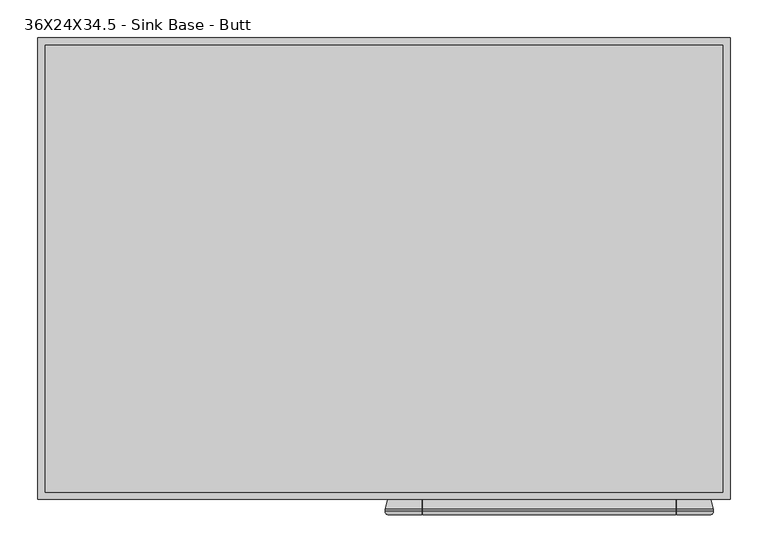
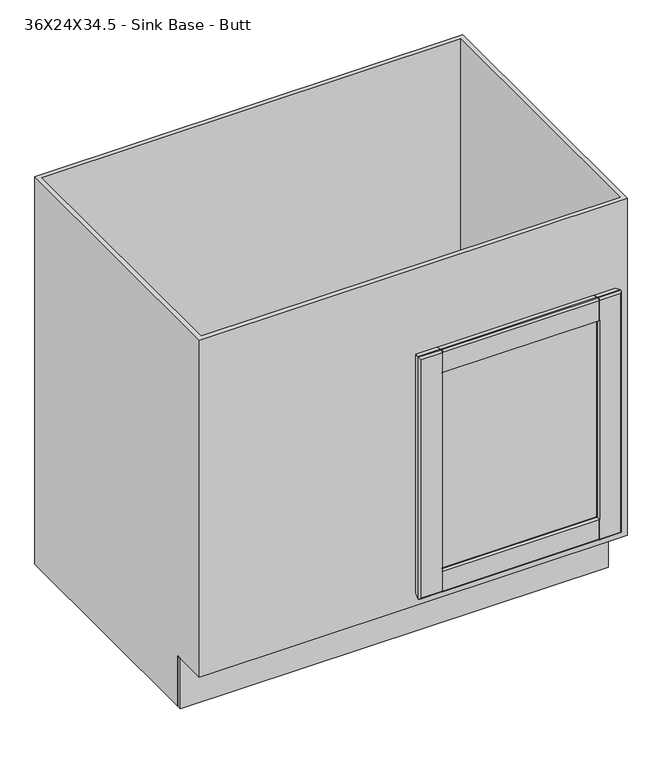
"""IFC4 building model written with IfcOpenShell, lengths in millimetres: furniture geometry, Cabinet-Base-Merillat-Double_Door-Marlin : 36X24X34.5 - Sink Base - Butt."""

import ifcopenshell
import ifcopenshell.guid

model = None  # the IFC model being written
_history = None  # IfcOwnerHistory: only IFC2X3 demands one
_inside = {}  # id of a spatial element -> (the spatial element, [elements in it])
_under = {}  # id of a project, library or spatial element -> (it, [spatial elements below it])
_declared = {}  # id of a project -> (the project, [libraries it declares])
_typed = {}  # id of a type object -> (the type object, [elements of that type])
_made_of = {}  # id of a material, layer set ... -> (it, [elements and type objects made of it])


def new_model(schema):
    """Start an empty IFC model of exactly this schema.

    Asked for "IFC4X3", IfcOpenShell would pick the latest addendum, in which some entities
    have other attributes; the version numbers below select the first issue.
    IFC2X3 requires an IfcOwnerHistory on every rooted entity: one is made here for all.
    """
    global model, _history
    if schema == "IFC4X3":
        model = ifcopenshell.file(schema_version=(4, 3, 0, 0))
    else:
        model = ifcopenshell.file(schema=schema)
    _inside.clear()
    _under.clear()
    _declared.clear()
    _typed.clear()
    _made_of.clear()
    _history = None
    if model.schema == "IFC2X3":
        org = make("IfcOrganization", Name="unknown")
        user = make(
            "IfcPersonAndOrganization",
            ThePerson=make("IfcPerson", FamilyName="unknown"),
            TheOrganization=org,
        )
        app = make(
            "IfcApplication",
            ApplicationDeveloper=org,
            Version="unknown",
            ApplicationFullName="unknown",
            ApplicationIdentifier="unknown",
        )
        _history = make(
            "IfcOwnerHistory",
            OwningUser=user,
            OwningApplication=app,
            ChangeAction="ADDED",
            CreationDate=0,
        )
    return model


def make(cls, **values):
    """One entity of the class cls with the attributes given. An attribute that is None is left unset."""
    return model.create_entity(
        cls, **{name: value for name, value in values.items() if value is not None}
    )


def rooted(cls, **values):
    """An entity with a GlobalId (a new one), such as an element, a storey or a relation."""
    return make(cls, GlobalId=ifcopenshell.guid.new(), OwnerHistory=_history, **values)


def si_unit(unit_type, name, prefix=None):
    """IfcSIUnit, for example si_unit("LENGTHUNIT", "METRE", prefix="MILLI")."""
    return make("IfcSIUnit", UnitType=unit_type, Prefix=prefix, Name=name)


def assignment(units):
    """IfcUnitAssignment: the units of a project."""
    return None if units is None else make("IfcUnitAssignment", Units=units)


def point(xyz):
    """IfcCartesianPoint."""
    return None if xyz is None else make("IfcCartesianPoint", Coordinates=xyz)


def direction(xyz):
    """IfcDirection."""
    return None if xyz is None else make("IfcDirection", DirectionRatios=xyz)


def frame(location, z_axis=None, x_axis=None):
    """IfcAxis2Placement3D, a coordinate frame: its origin and axes. An axis left out is left unset."""
    return make(
        "IfcAxis2Placement3D",
        Location=point(location),
        Axis=direction(z_axis),
        RefDirection=direction(x_axis),
    )


def origin():
    """The frame at (0, 0, 0) with its axes left unset."""
    return frame((0.0, 0.0, 0.0))


def origin_with_axes():
    """The frame at (0, 0, 0) with the z axis (0, 0, 1) and the x axis (1, 0, 0) written out."""
    return frame((0.0, 0.0, 0.0), z_axis=(0.0, 0.0, 1.0), x_axis=(1.0, 0.0, 0.0))


def place(relative_to, where):
    """IfcLocalPlacement: puts the frame where relative to a parent placement (None: the world)."""
    return make(
        "IfcLocalPlacement", PlacementRelTo=relative_to, RelativePlacement=where
    )


def context(
    kind, dimensions, precision=None, world=None, true_north=None, identifier=None
):
    """IfcGeometricRepresentationContext, for example the 3D "Model" context."""
    return make(
        "IfcGeometricRepresentationContext",
        ContextIdentifier=identifier,
        ContextType=kind,
        CoordinateSpaceDimension=dimensions,
        Precision=precision,
        WorldCoordinateSystem=world,
        TrueNorth=true_north,
    )


def project(units=None, contexts=None):
    """IfcProject with its units and contexts."""
    return rooted(
        "IfcProject",
        Name="project",
        RepresentationContexts=contexts,
        UnitsInContext=assignment(units),
    )


def spatial(cls, under=None, at=None, **own):
    """A site, building, storey or space (cls), placed at a placement, below another one or the project."""
    s = rooted(cls, ObjectPlacement=at, **own)
    if under is not None:
        _under.setdefault(under.id(), (under, []))[1].append(s)
    return s


def polyline(points):
    """IfcPolyline through the points."""
    return make("IfcPolyline", Points=[point(p) for p in points])


def circle_curve(where, radius):
    """IfcCircle in the frame where."""
    return make("IfcCircle", Position=where, Radius=radius)


def ellipse_curve(where, semi_axis1, semi_axis2):
    """IfcEllipse in the frame where."""
    return make(
        "IfcEllipse", Position=where, SemiAxis1=semi_axis1, SemiAxis2=semi_axis2
    )


def outline(outer, holes=None, kind="AREA"):
    """IfcArbitraryClosedProfileDef: a profile drawn as a closed curve; with holes, ...WithVoids."""
    if holes is None:
        return make("IfcArbitraryClosedProfileDef", ProfileType=kind, OuterCurve=outer)
    return make(
        "IfcArbitraryProfileDefWithVoids",
        ProfileType=kind,
        OuterCurve=outer,
        InnerCurves=holes,
    )


def extrude(swept, where, along, depth):
    """IfcExtrudedAreaSolid: the profile swept, set in the frame where, extruded along a direction by depth."""
    return make(
        "IfcExtrudedAreaSolid",
        SweptArea=swept,
        Position=where,
        ExtrudedDirection=direction(along),
        Depth=depth,
    )


def faces_of(points, faces, orient=None, outer=None):
    """IfcFace entities. A face is a list of loops; a loop is a list of indices into points, from 0.

    orient and outer hold one flag for each loop. By default every Orientation is true, the
    first loop of a face is its IfcFaceOuterBound and the others are IfcFaceBound.
    """
    made = []
    for i, loops in enumerate(faces):
        bounds = []
        for j, loop in enumerate(loops):
            is_outer = j == 0 if outer is None else outer[i][j]
            bounds.append(
                make(
                    "IfcFaceOuterBound" if is_outer else "IfcFaceBound",
                    Bound=make("IfcPolyLoop", Polygon=[points[k] for k in loop]),
                    Orientation=True if orient is None else orient[i][j],
                )
            )
        made.append(make("IfcFace", Bounds=bounds))
    return made


def faceted_brep(points, faces, orient=None, outer=None, voids=None):
    """IfcFacetedBrep: a solid bounded by flat faces; with voids (closed shells), ...WithVoids."""
    shared = [point(p) for p in points]
    hull = make("IfcClosedShell", CfsFaces=faces_of(shared, faces, orient, outer))
    if voids is None:
        return make("IfcFacetedBrep", Outer=hull)
    return make(
        "IfcFacetedBrepWithVoids",
        Outer=hull,
        Voids=[
            make(cls, CfsFaces=faces_of(shared, fs, o, b)) for cls, fs, o, b in voids
        ],
    )


def shape(context_of_items, identifier, shape_type, items):
    """IfcShapeRepresentation: the items that make up one representation, for example the "Body"."""
    return make(
        "IfcShapeRepresentation",
        ContextOfItems=context_of_items,
        RepresentationIdentifier=identifier,
        RepresentationType=shape_type,
        Items=items,
    )


def source(mapping_origin, context_of_items, identifier, shape_type, items):
    """IfcRepresentationMap: a shape defined once, which mapped items show again and again."""
    return make(
        "IfcRepresentationMap",
        MappingOrigin=mapping_origin,
        MappedRepresentation=shape(context_of_items, identifier, shape_type, items),
    )


def transform(
    local_origin,
    x_axis=None,
    y_axis=None,
    z_axis=None,
    scale=None,
    scale2=None,
    scale3=None,
    uniform=True,
):
    """IfcCartesianTransformationOperator3D, or its non-uniform kind. x_axis, y_axis, z_axis: its Axis1, 2, 3."""
    if uniform:
        return make(
            "IfcCartesianTransformationOperator3D",
            Axis1=direction(x_axis),
            Axis2=direction(y_axis),
            LocalOrigin=point(local_origin),
            Scale=scale,
            Axis3=direction(z_axis),
        )
    return make(
        "IfcCartesianTransformationOperator3DnonUniform",
        Axis1=direction(x_axis),
        Axis2=direction(y_axis),
        LocalOrigin=point(local_origin),
        Scale=scale,
        Axis3=direction(z_axis),
        Scale2=scale2,
        Scale3=scale3,
    )


def mapped(mapping_source, mapping_target):
    """IfcMappedItem: shows the shape of a source again, moved by a transform."""
    return make(
        "IfcMappedItem", MappingSource=mapping_source, MappingTarget=mapping_target
    )


def made_of(thing, what):
    """Note that an element or type object is made of a material, layer set ...; save() writes the relation."""
    if what is not None:
        _made_of.setdefault(what.id(), (what, []))[1].append(thing)
    return thing


def element(
    cls,
    number,
    at=None,
    inside=None,
    cuts=None,
    type_object=None,
    material=None,
    context=None,
    identifier="Body",
    shape_type=None,
    held_by="IfcProductDefinitionShape",
    body=None,
    shapes=None,
    **own,
):
    """One element of the class cls, such as IfcWall. Its Tag is "e" and its number.

    at: its placement. inside: the storey or other place that contains it. cuts: it is an
    opening in that element (IfcRelVoidsElement). A single representation is given by context,
    identifier, shape_type and body (its items); several are given by shapes. held_by: the class
    of the entity that holds the representations. save() writes the other relations.
    """
    e = rooted(cls, Tag="e%d" % number, ObjectPlacement=at, **own)
    if body is not None:
        shapes = [shape(context, identifier, shape_type, body)]
    if shapes is not None:
        e.Representation = make(held_by, Representations=shapes)
    if inside is not None:
        _inside.setdefault(inside.id(), (inside, []))[1].append(e)
    if cuts is not None:
        rooted(
            "IfcRelVoidsElement", RelatingBuildingElement=cuts, RelatedOpeningElement=e
        )
    if type_object is not None:
        _typed.setdefault(type_object.id(), (type_object, []))[1].append(e)
    return made_of(e, material)


def aggregate(whole, parts):
    """IfcRelAggregates: a whole, such as a stair, and the parts it consists of."""
    return rooted("IfcRelAggregates", RelatingObject=whole, RelatedObjects=parts)


def save(model, path):
    """Write the relations noted so far, then the file.

    IfcRelAggregates (storeys below a building ...), IfcRelContainedInSpatialStructure (elements
    in a storey), IfcRelDefinesByType, IfcRelAssociatesMaterial and IfcRelDeclares: one each for
    every whole, place, type object, material and project.
    """
    for whole, parts in _under.values():
        aggregate(whole, parts)
    for where, things in _inside.values():
        rooted(
            "IfcRelContainedInSpatialStructure",
            RelatedElements=things,
            RelatingStructure=where,
        )
    for kind, things in _typed.values():
        rooted("IfcRelDefinesByType", RelatedObjects=things, RelatingType=kind)
    for what, things in _made_of.values():
        rooted("IfcRelAssociatesMaterial", RelatedObjects=things, RelatingMaterial=what)
    for by, libraries in _declared.values():
        rooted("IfcRelDeclares", RelatingContext=by, RelatedDefinitions=libraries)
    model.write(path)


def plane_surface(at):
    """IfcPlane: the flat surface through the origin of the frame at, square to its z axis."""
    return make("IfcPlane", Position=at)


def cylinder_surface(at, radius):
    """IfcCylindricalSurface: all points at the distance radius from the z axis of the frame at."""
    return make("IfcCylindricalSurface", Position=at, Radius=radius)


def advanced_brep(points, edges, surfaces, faces):
    """IfcAdvancedBrep: a solid bounded by faces that lie on surfaces and meet in shared edges.

    An edge is (start, end): straight between two places in points (the first is 0);
    or (start, end, curve); or (start, end, curve, False) where it runs against its curve.
    A face is (place in surfaces, loops), or (place, loops, False) where it looks against
    its surface's normal. A loop lists edges by number (the first is 1), with a minus sign
    where the edge is run from its end to its start. The first loop is the outer one.
    """
    corners = [point(p) for p in points]
    vertices = [make("IfcVertexPoint", VertexGeometry=c) for c in corners]
    made = []
    for start, end, *more in edges:
        made.append(
            make(
                "IfcEdgeCurve",
                EdgeStart=vertices[start],
                EdgeEnd=vertices[end],
                EdgeGeometry=more[0] if more else make("IfcPolyline", Points=[corners[start], corners[end]]),
                SameSense=more[1] if len(more) > 1 else True,
            )
        )
    hull = []
    for where, loops, *sense in faces:
        bounds = []
        for j, loop in enumerate(loops):
            ring = [make("IfcOrientedEdge", EdgeElement=made[abs(k) - 1], Orientation=k > 0) for k in loop]
            bounds.append(
                make(
                    "IfcFaceOuterBound" if j == 0 else "IfcFaceBound",
                    Bound=make("IfcEdgeLoop", EdgeList=ring),
                    Orientation=True,
                )
            )
        hull.append(make("IfcAdvancedFace", Bounds=bounds, FaceSurface=surfaces[where], SameSense=sense[0] if sense else True))
    return make("IfcAdvancedBrep", Outer=make("IfcClosedShell", CfsFaces=hull))


def furniture_36x24x34_5_sink_base_butt_f9e5757f(model_context):
    return source(origin(), model_context, "Body", "SolidModel", [
        advanced_brep(
        [(453.7127049, -625.4496, 685.8), (450.6162124, -629.92, 682.7035075), (450.6162124, -629.92, 142.7964925), (453.7127049, -625.4496, 139.7), (453.7127049, -622.681, 139.7), (453.7127049, -622.681, 685.8), (450.2075049, -609.6, 143.2052), (450.2075049, -609.6, 682.2948), (405.5115422, -609.6, 637.5988372), (405.5115422, -609.6, 187.9011628), (405.1414105, -610.39375, 188.2712945), (403.0602514, -614.85681, 190.3524535), (403.0602514, -614.85681, 635.1475465), (405.1414105, -610.39375, 637.2287055), (404.4600209, -617.0969093, 188.952684), (404.4600209, -617.0969093, 636.547316), (418.7877049, -617.347, 174.625), (418.7877049, -617.347, 650.875), (418.7877049, -622.173, 174.625), (418.7877049, -622.173, 650.875), (404.4600209, -622.4230907, 188.952684), (404.4600209, -622.4230907, 636.547316), (403.0602514, -624.66319, 190.3524535), (403.0602514, -624.66319, 635.1475465), (405.1414105, -629.12625, 188.2712945), (405.5086747, -629.9138508, 187.9040302), (405.5115422, -629.92, 637.5988372), (405.1414105, -629.12625, 637.2287055), (405.5086747, -629.92, 142.7964925), (405.5086747, -625.4496, 139.7), (23.4216974, -629.92, 142.7964925), (20.3252049, -625.4496, 139.7), (68.4894236, -625.4496, 139.7), (68.4894236, -629.92, 142.7964925), (403.9211747, -625.4496, 139.7), (403.9211747, -629.92, 142.7964925), (70.0769236, -629.92, 142.7964925), (70.0769236, -625.4496, 139.7), (405.5086747, -622.681, 139.7), (20.3252049, -622.681, 139.7), (68.4894236, -622.681, 139.7), (403.9211747, -622.681, 139.7), (70.0769236, -622.681, 139.7), (405.5086747, -609.6, 143.2052), (23.8304049, -609.6, 143.2052), (68.4894236, -609.6, 143.2052), (403.9211747, -609.6, 143.2052), (70.0769236, -609.6, 143.2052), (70.9776584, -614.85681, 190.3524535), (403.9211747, -610.39375, 188.2712945), (403.9211747, -609.6, 187.9011628), (70.0769236, -609.6, 187.9011628), (70.0769236, -610.39375, 188.2712945), (68.8964994, -610.39375, 188.2712945), (69.577889, -617.0969093, 188.952684), (55.2502049, -617.347, 174.625), (55.2502049, -622.173, 174.625), (69.577889, -622.4230907, 188.952684), (70.9776584, -624.66319, 190.3524535), (68.8964994, -629.12625, 188.2712945), (70.0769236, -629.12625, 188.2712945), (70.0769236, -629.92, 187.9011628), (403.9211747, -629.92, 187.9011628), (403.9211747, -629.12625, 188.2712945), (23.4216974, -629.92, 682.7035075), (20.3252049, -625.4496, 685.8), (20.3252049, -622.681, 685.8), (23.8304049, -609.6, 682.2948), (68.5263677, -609.6, 187.9011628), (68.5263677, -609.6, 637.5988372), (68.8964994, -610.39375, 637.2287055), (70.9776584, -614.85681, 635.1475465), (69.577889, -617.0969093, 636.547316), (55.2502049, -617.347, 650.875), (55.2502049, -622.173, 650.875), (69.577889, -622.4230907, 636.547316), (70.9776584, -624.66319, 635.1475465), (68.8964994, -629.12625, 637.2287055), (68.5263677, -629.92, 637.5988372), (68.5263677, -629.92, 187.9011628), (68.4894236, -629.92, 682.7035075), (68.4894236, -625.4496, 685.8), (405.5086747, -625.4496, 685.8), (405.5086747, -629.92, 682.7035075), (70.0769236, -625.4496, 685.8), (70.0769236, -629.92, 682.7035075), (403.9211747, -629.92, 682.7035075), (403.9211747, -625.4496, 685.8), (68.4894236, -622.681, 685.8), (405.5086747, -622.681, 685.8), (70.0769236, -622.681, 685.8), (403.9211747, -622.681, 685.8), (68.4894236, -609.6, 682.2948), (405.5086747, -609.6, 682.2948), (70.0769236, -609.6, 682.2948), (403.9211747, -609.6, 682.2948), (70.0769236, -609.6, 637.5988372), (403.9211747, -609.6, 637.5988372), (70.0769236, -610.39375, 637.2287055), (403.9211747, -610.39375, 637.2287055), (403.9211747, -629.12625, 637.2287055), (403.9211747, -629.92, 637.5988372), (70.0769236, -629.92, 637.5988372), (70.0769236, -629.12625, 637.2287055), (70.0769236, -610.39375, 681.6857412), (70.0769236, -622.7855037, 685.00625), (70.0769236, -625.4496, 685.00625), (70.0769236, -629.12625, 682.5526052), (68.4894236, -629.12625, 637.2287055), (68.4894236, -629.12625, 682.5526052), (68.4894236, -625.4496, 685.00625), (68.4894236, -622.7855037, 685.00625), (68.4894236, -610.39375, 681.6857412), (68.4894236, -610.39375, 637.2287055), (405.5086747, -610.39375, 637.2287055), (405.5086747, -610.39375, 681.6857412), (405.5086747, -622.7855037, 685.00625), (405.5086747, -625.4496, 685.00625), (405.5086747, -629.12625, 682.5526052), (405.5086747, -629.12625, 637.2287055), (403.9211747, -629.12625, 682.5526052), (403.9211747, -625.4496, 685.00625), (403.9211747, -622.7855037, 685.00625), (403.9211747, -610.39375, 681.6857412), (405.5086747, -629.12625, 188.2712945), (405.5086747, -629.12625, 142.9473948), (405.5086747, -625.4496, 140.49375), (405.5086747, -622.7855037, 140.49375), (405.5086747, -610.39375, 143.8142588), (405.5086747, -610.39375, 188.2712945), (403.9211747, -610.39375, 143.8142588), (403.9211747, -622.7855037, 140.49375), (403.9211747, -625.4496, 140.49375), (403.9211747, -629.12625, 142.9473948), (70.0769236, -629.12625, 142.9473948), (70.0769236, -625.4496, 140.49375), (70.0769236, -622.7855037, 140.49375), (70.0769236, -610.39375, 143.8142588), (68.4894236, -629.12625, 188.2712945), (68.4894236, -610.39375, 188.2712945), (68.4894236, -610.39375, 143.8142588), (68.4894236, -622.7855037, 140.49375), (68.4894236, -625.4496, 140.49375), (68.4894236, -629.12625, 142.9473948)],
        [
            (0, 1, ellipse_curve(frame((448.9375049, -625.4496, 681.0248), z_axis=(0.7071067811865475, 0.0, -0.7071067811865475), x_axis=(0.7071067811865474, 0.0, 0.7071067811865476)), 6.7531526, 4.7752)),
            (1, 2),
            (2, 3, ellipse_curve(frame((448.9375049, -625.4496, 144.4752), z_axis=(0.7071067811865475, 0.0, 0.7071067811865475), x_axis=(-0.7071067811865474, 0.0, 0.7071067811865476)), 6.7531526, 4.7752)),
            (3, 0),
            (3, 4),
            (4, 5),
            (5, 0),
            (4, 6),
            (6, 7),
            (7, 5),
            (8, 9),
            (9, 10),
            (10, 11),
            (11, 12),
            (12, 13),
            (13, 8),
            (11, 14, ellipse_curve(frame((404.4875049, -615.5223492, 188.9252), z_axis=(0.7071067811865475, 0.0, 0.7071067811865475), x_axis=(-0.7071067811865474, 0.0, 0.7071067811865476)), 2.2271035, 1.5748)),
            (14, 15),
            (15, 12, ellipse_curve(frame((404.4875049, -615.5223492, 636.5748), z_axis=(0.7071067811865475, 0.0, -0.7071067811865475), x_axis=(0.7071067811865474, 0.0, 0.7071067811865476)), 2.2271035, 1.5748)),
            (14, 16),
            (16, 17),
            (17, 15),
            (16, 18),
            (18, 19),
            (19, 17),
            (18, 20),
            (20, 21),
            (21, 19),
            (20, 22, ellipse_curve(frame((404.4875049, -623.9976508, 188.9252), z_axis=(0.7071067811865475, 0.0, 0.7071067811865475), x_axis=(-0.7071067811865474, 0.0, 0.7071067811865476)), 2.2271035, 1.5748)),
            (22, 23),
            (23, 21, ellipse_curve(frame((404.4875049, -623.9976508, 636.5748), z_axis=(0.7071067811865475, 0.0, -0.7071067811865475), x_axis=(0.7071067811865474, 0.0, 0.7071067811865476)), 2.2271035, 1.5748)),
            (22, 24),
            (24, 25),
            (25, 26),
            (26, 27),
            (27, 23),
            (2, 28),
            (28, 29, circle_curve(frame((405.5086747, -625.4496, 144.4752), z_axis=(1.0, 0.0, 0.0), x_axis=(0.0, 1.0, 0.0)), 4.7752)),
            (29, 3),
            (30, 31, ellipse_curve(frame((25.1004049, -625.4496, 144.4752), z_axis=(0.7071067811865475, 0.0, -0.7071067811865475), x_axis=(0.7071067811865476, 0.0, 0.7071067811865474)), 6.7531526, 4.7752)),
            (31, 32),
            (32, 33, circle_curve(frame((68.4894236, -625.4496, 144.4752), z_axis=(-1.0, 0.0, 0.0), x_axis=(0.0, 1.0, 0.0)), 4.7752)),
            (33, 30),
            (34, 35, circle_curve(frame((403.9211747, -625.4496, 144.4752), z_axis=(-1.0, 0.0, 0.0), x_axis=(0.0, 1.0, 0.0)), 4.7752)),
            (35, 36),
            (36, 37, circle_curve(frame((70.0769236, -625.4496, 144.4752), z_axis=(1.0, 0.0, 0.0), x_axis=(0.0, 1.0, 0.0)), 4.7752)),
            (37, 34),
            (29, 38),
            (38, 4),
            (31, 39),
            (39, 40),
            (40, 32),
            (41, 34),
            (37, 42),
            (42, 41),
            (38, 43),
            (43, 6),
            (39, 44),
            (44, 45),
            (45, 40),
            (46, 41),
            (42, 47),
            (47, 46),
            (48, 11),
            (10, 49),
            (49, 50),
            (50, 51),
            (51, 52),
            (52, 53),
            (53, 48),
            (48, 54, ellipse_curve(frame((69.5504049, -615.5223492, 188.9252), z_axis=(0.7071067811865475, 0.0, -0.7071067811865475), x_axis=(0.7071067811865476, 0.0, 0.7071067811865474)), 2.2271035, 1.5748)),
            (54, 14),
            (54, 55),
            (55, 16),
            (55, 56),
            (56, 18),
            (56, 57),
            (57, 20),
            (57, 58, ellipse_curve(frame((69.5504049, -623.9976508, 188.9252), z_axis=(0.7071067811865475, 0.0, -0.7071067811865475), x_axis=(0.7071067811865476, 0.0, 0.7071067811865474)), 2.2271035, 1.5748)),
            (58, 22),
            (58, 59),
            (59, 60),
            (60, 61),
            (61, 62),
            (62, 63),
            (63, 24),
            (30, 64),
            (64, 65, ellipse_curve(frame((25.1004049, -625.4496, 681.0248), z_axis=(-0.7071067811865475, 0.0, -0.7071067811865475), x_axis=(0.7071067811865474, 0.0, -0.7071067811865476)), 6.7531526, 4.7752)),
            (65, 31),
            (65, 66),
            (66, 39),
            (66, 67),
            (67, 44),
            (68, 69),
            (69, 70),
            (70, 71),
            (71, 48),
            (53, 68),
            (71, 72, ellipse_curve(frame((69.5504049, -615.5223492, 636.5748), z_axis=(-0.7071067811865475, 0.0, -0.7071067811865475), x_axis=(0.7071067811865474, 0.0, -0.7071067811865476)), 2.2271035, 1.5748)),
            (72, 54),
            (72, 73),
            (73, 55),
            (73, 74),
            (74, 56),
            (74, 75),
            (75, 57),
            (75, 76, ellipse_curve(frame((69.5504049, -623.9976508, 636.5748), z_axis=(-0.7071067811865475, 0.0, -0.7071067811865475), x_axis=(0.7071067811865474, 0.0, -0.7071067811865476)), 2.2271035, 1.5748)),
            (76, 58),
            (76, 77),
            (77, 78),
            (78, 79),
            (79, 59),
            (64, 80),
            (80, 81, circle_curve(frame((68.4894236, -625.4496, 681.0248), z_axis=(-1.0, 0.0, 0.0), x_axis=(0.0, 1.0, 0.0)), 4.7752)),
            (81, 65),
            (0, 82),
            (82, 83, circle_curve(frame((405.5086747, -625.4496, 681.0248), z_axis=(1.0, 0.0, 0.0), x_axis=(0.0, 1.0, 0.0)), 4.7752)),
            (83, 1),
            (84, 85, circle_curve(frame((70.0769236, -625.4496, 681.0248), z_axis=(1.0, 0.0, 0.0), x_axis=(0.0, 1.0, 0.0)), 4.7752)),
            (85, 86),
            (86, 87, circle_curve(frame((403.9211747, -625.4496, 681.0248), z_axis=(-1.0, 0.0, 0.0), x_axis=(0.0, 1.0, 0.0)), 4.7752)),
            (87, 84),
            (81, 88),
            (88, 66),
            (5, 89),
            (89, 82),
            (90, 84),
            (87, 91),
            (91, 90),
            (88, 92),
            (92, 67),
            (7, 93),
            (93, 89),
            (94, 90),
            (91, 95),
            (95, 94),
            (43, 9),
            (8, 93),
            (92, 69),
            (68, 45),
            (96, 94),
            (95, 97),
            (97, 96),
            (50, 46),
            (47, 51),
            (12, 71),
            (70, 98),
            (98, 96),
            (97, 99),
            (99, 13),
            (15, 72),
            (17, 73),
            (19, 74),
            (21, 75),
            (23, 76),
            (27, 100),
            (100, 101),
            (101, 102),
            (102, 103),
            (103, 77),
            (83, 26),
            (25, 28),
            (33, 79),
            (78, 80),
            (85, 102),
            (101, 86),
            (35, 62),
            (61, 36),
            (98, 104),
            (104, 105),
            (105, 106),
            (106, 107, circle_curve(frame((70.0769236, -625.4496, 681.0248), z_axis=(1.0, 0.0, 0.0), x_axis=(0.0, 0.0, 1.0)), 3.98145)),
            (107, 103),
            (78, 108),
            (108, 109),
            (109, 110, circle_curve(frame((68.4894236, -625.4496, 681.0248), z_axis=(-1.0, 0.0, 0.0), x_axis=(0.0, 0.0, 1.0)), 3.98145)),
            (110, 111),
            (111, 112),
            (112, 113),
            (113, 69),
            (77, 108),
            (107, 109),
            (106, 110),
            (105, 111),
            (104, 112),
            (70, 113),
            (8, 114),
            (114, 115),
            (115, 116),
            (116, 117),
            (117, 118, circle_curve(frame((405.5086747, -625.4496, 681.0248), z_axis=(1.0, 0.0, 0.0), x_axis=(0.0, 0.0, 1.0)), 3.98145)),
            (118, 119),
            (119, 26),
            (100, 120),
            (120, 121, circle_curve(frame((403.9211747, -625.4496, 681.0248), z_axis=(-1.0, 0.0, 0.0), x_axis=(0.0, 0.0, 1.0)), 3.98145)),
            (121, 122),
            (122, 123),
            (123, 99),
            (119, 27),
            (118, 120),
            (117, 121),
            (116, 122),
            (115, 123),
            (114, 13),
            (25, 124),
            (124, 125),
            (125, 126, circle_curve(frame((405.5086747, -625.4496, 144.4752), z_axis=(1.0, 0.0, 0.0), x_axis=(0.0, 0.0, 1.0)), 3.98145)),
            (126, 127),
            (127, 128),
            (128, 129),
            (129, 9),
            (49, 130),
            (130, 131),
            (131, 132),
            (132, 133, circle_curve(frame((403.9211747, -625.4496, 144.4752), z_axis=(-1.0, 0.0, 0.0), x_axis=(0.0, 0.0, 1.0)), 3.98145)),
            (133, 63),
            (129, 10),
            (128, 130),
            (127, 131),
            (126, 132),
            (125, 133),
            (124, 24),
            (60, 134),
            (134, 135, circle_curve(frame((70.0769236, -625.4496, 144.4752), z_axis=(1.0, 0.0, 0.0), x_axis=(0.0, 0.0, 1.0)), 3.98145)),
            (135, 136),
            (136, 137),
            (137, 52),
            (138, 79),
            (68, 139),
            (139, 140),
            (140, 141),
            (141, 142),
            (142, 143, circle_curve(frame((68.4894236, -625.4496, 144.4752), z_axis=(-1.0, 0.0, 0.0), x_axis=(0.0, 0.0, 1.0)), 3.98145)),
            (143, 138),
            (138, 59),
            (53, 139),
            (137, 140),
            (136, 141),
            (135, 142),
            (134, 143),
        ],
        [
            cylinder_surface(frame((448.9375049, -625.4496, 685.8), z_axis=(0.0, 0.0, 1.0), x_axis=(0.0, 1.0, 0.0)), 4.7752),
            plane_surface(frame((453.7127049, -625.4496, 685.8), z_axis=(1.0, 0.0, 0.0), x_axis=(0.0, 0.0, -1.0))),
            plane_surface(frame((453.7127049, -622.681, 685.8), z_axis=(0.9659229350723619, 0.25882983502910506, 0.0), x_axis=(0.0, 0.0, -1.0))),
            plane_surface(frame((405.5115422, -609.6, 637.5988372), z_axis=(-0.9063077870366099, 0.4226182617407856, 0.0), x_axis=(0.0, 0.0, -1.0))),
            cylinder_surface(frame((404.4875049, -615.5223492, 685.8), z_axis=(0.0, 0.0, 1.0000000000000002), x_axis=(-0.01745240643729364, -0.9998476951563912, 0.0)), 1.5748),
            plane_surface(frame((404.4600209, -617.0969093, 636.547316), z_axis=(-0.017452406437322144, -0.9998476951563906, 0.0), x_axis=(0.0, 0.0, -1.0))),
            plane_surface(frame((418.7877049, -617.347, 650.875), z_axis=(-1.0, 0.0, 0.0), x_axis=(0.0, 0.0, -1.0))),
            plane_surface(frame((418.7877049, -622.173, 650.875), z_axis=(-0.01745240643727848, 0.9998476951563914, 0.0), x_axis=(0.0, 0.0, -1.0))),
            cylinder_surface(frame((404.4875049, -623.9976508, 685.8), z_axis=(0.0, 0.0, 1.0000000000000002), x_axis=(-0.9063077870367326, -0.42261826174052236, 0.0)), 1.5748),
            plane_surface(frame((403.0602514, -624.66319, 635.1475465), z_axis=(-0.9063077870366333, -0.4226182617407352, 0.0), x_axis=(0.0, 0.0, -1.0))),
            cylinder_surface(frame((453.7127049, -625.4496, 144.4752), z_axis=(1.0, 0.0, 0.0), x_axis=(0.0, 1.0, 0.0)), 4.7752),
            plane_surface(frame((453.7127049, -625.4496, 139.7), z_axis=(0.0, 0.0, -1.0), x_axis=(-1.0, 0.0, 0.0))),
            plane_surface(frame((453.7127049, -622.681, 139.7), z_axis=(0.0, 0.25882983502910506, -0.9659229350723619), x_axis=(-1.0, 0.0, 0.0))),
            plane_surface(frame((405.5115422, -609.6, 187.9011628), z_axis=(0.0, 0.4226182617407856, 0.9063077870366099), x_axis=(-1.0, 0.0, 0.0))),
            cylinder_surface(frame((453.7127049, -615.5223492, 188.9252), z_axis=(1.0000000000000002, 0.0, 0.0), x_axis=(0.0, -0.9998476951563912, 0.01745240643729364)), 1.5748),
            plane_surface(frame((404.4600209, -617.0969093, 188.952684), z_axis=(0.0, -0.9998476951563906, 0.017452406437322144), x_axis=(-1.0, 0.0, 0.0))),
            plane_surface(frame((418.7877049, -617.347, 174.625), z_axis=(0.0, 0.0, 1.0), x_axis=(-1.0, 0.0, 0.0))),
            plane_surface(frame((418.7877049, -622.173, 174.625), z_axis=(0.0, 0.9998476951563914, 0.01745240643727848), x_axis=(-1.0, 0.0, 0.0))),
            cylinder_surface(frame((453.7127049, -623.9976508, 188.9252), z_axis=(1.0000000000000002, 0.0, 0.0), x_axis=(0.0, -0.42261826174052236, 0.9063077870367326)), 1.5748),
            plane_surface(frame((403.0602514, -624.66319, 190.3524535), z_axis=(0.0, -0.4226182617407352, 0.9063077870366333), x_axis=(-1.0, 0.0, 0.0))),
            cylinder_surface(frame((25.1004049, -625.4496, 139.7), z_axis=(0.0, 0.0, -1.0), x_axis=(0.0, 1.0, 0.0)), 4.7752),
            plane_surface(frame((20.3252049, -625.4496, 139.7), z_axis=(-1.0, 0.0, 0.0), x_axis=(0.0, 0.0, 1.0))),
            plane_surface(frame((20.3252049, -622.681, 139.7), z_axis=(-0.9659229350723619, 0.25882983502910506, 0.0), x_axis=(0.0, 0.0, 1.0))),
            plane_surface(frame((68.5263677, -609.6, 187.9011628), z_axis=(0.9063077870366099, 0.4226182617407856, 0.0), x_axis=(0.0, 0.0, 1.0))),
            cylinder_surface(frame((69.5504049, -615.5223492, 139.7), z_axis=(0.0, 0.0, -1.0000000000000002), x_axis=(0.01745240643729364, -0.9998476951563912, 0.0)), 1.5748),
            plane_surface(frame((69.577889, -617.0969093, 188.952684), z_axis=(0.017452406437322144, -0.9998476951563906, 0.0), x_axis=(0.0, 0.0, 1.0))),
            plane_surface(frame((55.2502049, -617.347, 174.625), z_axis=(1.0, 0.0, 0.0), x_axis=(0.0, 0.0, 1.0))),
            plane_surface(frame((55.2502049, -622.173, 174.625), z_axis=(0.01745240643727848, 0.9998476951563914, 0.0), x_axis=(0.0, 0.0, 1.0))),
            cylinder_surface(frame((69.5504049, -623.9976508, 139.7), z_axis=(0.0, 0.0, -1.0000000000000002), x_axis=(0.9063077870367326, -0.42261826174052236, 0.0)), 1.5748),
            plane_surface(frame((70.9776584, -624.66319, 190.3524535), z_axis=(0.9063077870366333, -0.4226182617407352, 0.0), x_axis=(0.0, 0.0, 1.0))),
            cylinder_surface(frame((20.3252049, -625.4496, 681.0248), z_axis=(-1.0, 0.0, 0.0), x_axis=(0.0, 1.0, 0.0)), 4.7752),
            plane_surface(frame((20.3252049, -625.4496, 685.8), z_axis=(0.0, 0.0, 1.0), x_axis=(1.0, 0.0, 0.0))),
            plane_surface(frame((20.3252049, -622.681, 685.8), z_axis=(0.0, 0.25882983502910506, 0.9659229350723619), x_axis=(1.0, 0.0, 0.0))),
            plane_surface(frame((23.8304049, -609.6, 682.2948), z_axis=(0.0, 1.0, 0.0), x_axis=(1.0, 0.0, 0.0))),
            plane_surface(frame((68.5263677, -609.6, 637.5988372), z_axis=(0.0, 0.4226182617407856, -0.9063077870366099), x_axis=(1.0, 0.0, 0.0))),
            cylinder_surface(frame((20.3252049, -615.5223492, 636.5748), z_axis=(-1.0000000000000002, 0.0, 0.0), x_axis=(0.0, -0.9998476951563912, -0.01745240643729364)), 1.5748),
            plane_surface(frame((69.577889, -617.0969093, 636.547316), z_axis=(0.0, -0.9998476951563906, -0.017452406437322144), x_axis=(1.0, 0.0, 0.0))),
            plane_surface(frame((55.2502049, -617.347, 650.875), z_axis=(0.0, 0.0, -1.0), x_axis=(1.0, 0.0, 0.0))),
            plane_surface(frame((55.2502049, -622.173, 650.875), z_axis=(0.0, 0.9998476951563914, -0.01745240643727848), x_axis=(1.0, 0.0, 0.0))),
            cylinder_surface(frame((20.3252049, -623.9976508, 636.5748), z_axis=(-1.0000000000000002, 0.0, 0.0), x_axis=(0.0, -0.42261826174052236, -0.9063077870367326)), 1.5748),
            plane_surface(frame((70.9776584, -624.66319, 635.1475465), z_axis=(0.0, -0.4226182617407352, -0.9063077870366333), x_axis=(1.0, 0.0, 0.0))),
            plane_surface(frame((68.5263677, -629.92, 637.5988372), z_axis=(0.0, -1.0, 0.0), x_axis=(1.0, 0.0, 0.0))),
            plane_surface(frame((70.0769236, -629.92, 637.5988372), z_axis=(-1.0, 0.0, 0.0), x_axis=(0.0, 0.906307787036771, -0.4226182617404399))),
            plane_surface(frame((68.4894236, -629.92, 637.5988372), z_axis=(1.0, 0.0, 0.0), x_axis=(0.0, -0.906307787036771, 0.4226182617404399))),
            plane_surface(frame((70.0769236, -629.92, 637.5988372), z_axis=(0.0, 0.4226182617404399, 0.906307787036771), x_axis=(-1.0, 0.0, 0.0))),
            plane_surface(frame((70.0769236, -629.12625, 637.2287055), z_axis=(0.0, -1.0, 0.0), x_axis=(-1.0, 0.0, 0.0))),
            cylinder_surface(frame((68.4894236, -625.4496, 681.0248), z_axis=(-1.0, 0.0, 0.0), x_axis=(0.0, 0.0, 1.0)), 3.98145),
            plane_surface(frame((70.0769236, -625.4496, 685.00625), z_axis=(0.0, 0.0, 1.0), x_axis=(-1.0, 0.0, 0.0))),
            plane_surface(frame((70.0769236, -622.7855037, 685.00625), z_axis=(0.0, 0.25882983502913415, 0.9659229350723542), x_axis=(-1.0, 0.0, 0.0))),
            plane_surface(frame((70.0769236, -610.39375, 681.6857412), z_axis=(0.0, 1.0, 0.0), x_axis=(-1.0, 0.0, 0.0))),
            plane_surface(frame((70.0769236, -610.39375, 637.2287055), z_axis=(0.0, -0.4226182617405111, 0.9063077870367379), x_axis=(-1.0, 0.0, 0.0))),
            plane_surface(frame((405.5086747, -629.92, 637.5988372), z_axis=(-1.0, 0.0, 0.0), x_axis=(0.0, 0.9063077870367783, -0.42261826174042444))),
            plane_surface(frame((403.9211747, -629.92, 637.5988372), z_axis=(1.0, 0.0, 0.0), x_axis=(0.0, -0.9063077870367783, 0.42261826174042444))),
            plane_surface(frame((405.5086747, -629.92, 637.5988372), z_axis=(0.0, 0.42261826174042444, 0.9063077870367783), x_axis=(-1.0, 0.0, 0.0))),
            plane_surface(frame((405.5086747, -629.12625, 637.2287055), z_axis=(0.0, -1.0, 0.0), x_axis=(-1.0, 0.0, 0.0))),
            cylinder_surface(frame((403.9211747, -625.4496, 681.0248), z_axis=(-1.0, 0.0, 0.0), x_axis=(0.0, 0.0, 1.0)), 3.98145),
            plane_surface(frame((405.5086747, -625.4496, 685.00625), z_axis=(0.0, 0.0, 1.0), x_axis=(-1.0, 0.0, 0.0))),
            plane_surface(frame((405.5086747, -622.7855037, 685.00625), z_axis=(0.0, 0.25882983502911566, 0.965922935072359), x_axis=(-1.0, 0.0, 0.0))),
            plane_surface(frame((405.5086747, -610.39375, 681.6857412), z_axis=(0.0, 1.0, 0.0), x_axis=(-1.0, 0.0, 0.0))),
            plane_surface(frame((405.5086747, -610.39375, 637.2287055), z_axis=(0.0, -0.42261826174056427, 0.9063077870367131), x_axis=(-1.0, 0.0, 0.0))),
            plane_surface(frame((405.5086747, -625.4496, 149.2504), z_axis=(-1.0, 0.0, 0.0), x_axis=(0.0, -1.0, 0.0))),
            plane_surface(frame((403.9211747, -625.4496, 149.2504), z_axis=(1.0, 0.0, 0.0), x_axis=(0.0, 1.0, 0.0))),
            plane_surface(frame((405.5086747, -609.6, 187.9011628), z_axis=(0.0, -0.42261826173999295, -0.9063077870369795), x_axis=(-1.0, 0.0, 0.0))),
            plane_surface(frame((405.5086747, -610.39375, 188.2712945), z_axis=(0.0, 1.0, 0.0), x_axis=(-1.0, 0.0, 0.0))),
            plane_surface(frame((405.5086747, -610.39375, 143.8142588), z_axis=(0.0, 0.2588298350290845, -0.9659229350723675), x_axis=(-1.0, 0.0, 0.0))),
            plane_surface(frame((405.5086747, -622.7855037, 140.49375), z_axis=(0.0, 0.0, -1.0), x_axis=(-1.0, 0.0, 0.0))),
            cylinder_surface(frame((403.9211747, -625.4496, 144.4752), z_axis=(-1.0, 0.0, 0.0), x_axis=(0.0, 0.0, 1.0)), 3.98145),
            plane_surface(frame((405.5086747, -629.12625, 142.9473948), z_axis=(0.0, -1.0, 0.0), x_axis=(-1.0, 0.0, 0.0))),
            plane_surface(frame((405.5086747, -629.12625, 188.2712945), z_axis=(0.0, 0.4226182617407698, -0.9063077870366172), x_axis=(-1.0, 0.0, 0.0))),
            plane_surface(frame((70.0769236, -629.12625, 188.2712945), z_axis=(-1.0, 0.0, 0.0), x_axis=(0.0, -0.906307787036583, -0.42261826174084305))),
            plane_surface(frame((68.4894236, -629.12625, 188.2712945), z_axis=(1.0, 0.0, 0.0), x_axis=(0.0, 0.906307787036583, 0.42261826174084305))),
            plane_surface(frame((70.0769236, -629.12625, 188.2712945), z_axis=(0.0, 0.42261826174084305, -0.906307787036583), x_axis=(-1.0, 0.0, 0.0))),
            plane_surface(frame((70.0769236, -609.6, 187.9011628), z_axis=(0.0, -0.42261826174073325, -0.9063077870366342), x_axis=(-1.0, 0.0, 0.0))),
            plane_surface(frame((70.0769236, -610.39375, 188.2712945), z_axis=(0.0, 1.0, 0.0), x_axis=(-1.0, 0.0, 0.0))),
            plane_surface(frame((70.0769236, -610.39375, 143.8142588), z_axis=(0.0, 0.2588298350290967, -0.9659229350723642), x_axis=(-1.0, 0.0, 0.0))),
            plane_surface(frame((70.0769236, -622.7855037, 140.49375), z_axis=(0.0, 0.0, -1.0), x_axis=(-1.0, 0.0, 0.0))),
            cylinder_surface(frame((68.4894236, -625.4496, 144.4752), z_axis=(-1.0, 0.0, 0.0), x_axis=(0.0, 0.0, 1.0)), 3.98145),
            plane_surface(frame((70.0769236, -629.12625, 142.9473948), z_axis=(0.0, -1.0, 0.0), x_axis=(-1.0, 0.0, 0.0))),
        ],
        [
            (0, [[1, 2, 3, 4]]),
            (1, [[-4, 5, 6, 7]]),
            (2, [[-6, 8, 9, 10]]),
            (3, [[11, 12, 13, 14, 15, 16]]),
            (4, [[-14, 17, 18, 19]]),
            (5, [[-18, 20, 21, 22]]),
            (6, [[-21, 23, 24, 25]]),
            (7, [[-24, 26, 27, 28]]),
            (8, [[-27, 29, 30, 31]]),
            (9, [[-30, 32, 33, 34, 35, 36]]),
            (10, [[-3, 37, 38, 39]]),
            (10, [[40, 41, 42, 43]]),
            (10, [[44, 45, 46, 47]]),
            (11, [[-5, -39, 48, 49]]),
            (11, [[50, 51, 52, -41]]),
            (11, [[53, -47, 54, 55]]),
            (12, [[-8, -49, 56, 57]]),
            (12, [[58, 59, 60, -51]]),
            (12, [[61, -55, 62, 63]]),
            (13, [[64, -13, 65, 66, 67, 68, 69, 70]]),
            (14, [[-17, -64, 71, 72]]),
            (15, [[-20, -72, 73, 74]]),
            (16, [[-23, -74, 75, 76]]),
            (17, [[-26, -76, 77, 78]]),
            (18, [[-29, -78, 79, 80]]),
            (19, [[-80, 81, 82, 83, 84, 85, 86, -32]]),
            (20, [[-40, 87, 88, 89]]),
            (21, [[-50, -89, 90, 91]]),
            (22, [[-58, -91, 92, 93]]),
            (23, [[94, 95, 96, 97, -70, 98]]),
            (24, [[-71, -97, 99, 100]]),
            (25, [[-73, -100, 101, 102]]),
            (26, [[-75, -102, 103, 104]]),
            (27, [[-77, -104, 105, 106]]),
            (28, [[-79, -106, 107, 108]]),
            (29, [[-108, 109, 110, 111, 112, -81]]),
            (30, [[-88, 113, 114, 115]]),
            (30, [[-1, 116, 117, 118]]),
            (30, [[119, 120, 121, 122]]),
            (31, [[-90, -115, 123, 124]]),
            (31, [[-7, 125, 126, -116]]),
            (31, [[127, -122, 128, 129]]),
            (32, [[-92, -124, 130, 131]]),
            (32, [[-10, 132, 133, -125]]),
            (32, [[134, -129, 135, 136]]),
            (33, [[-9, -57, 137, -11, 138, -132]]),
            (33, [[-93, -131, 139, -94, 140, -59]]),
            (33, [[141, -136, 142, 143]]),
            (33, [[144, -63, 145, -67]]),
            (34, [[146, -96, 147, 148, -143, 149, 150, -15]]),
            (35, [[-19, 151, -99, -146]]),
            (36, [[-22, 152, -101, -151]]),
            (37, [[-25, 153, -103, -152]]),
            (38, [[-28, 154, -105, -153]]),
            (39, [[-31, 155, -107, -154]]),
            (40, [[-155, -36, 156, 157, 158, 159, 160, -109]]),
            (41, [[-2, -118, 161, -34, 162, -37]]),
            (41, [[-87, -43, 163, -111, 164, -113]]),
            (41, [[165, -158, 166, -120]]),
            (41, [[167, -84, 168, -45]]),
            (42, [[169, 170, 171, 172, 173, -159, -165, -119, -127, -134, -141, -148]]),
            (43, [[174, 175, 176, 177, 178, 179, 180, -139, -130, -123, -114, -164]]),
            (44, [[-174, -110, 181]]),
            (45, [[-173, 182, -175, -181, -160]]),
            (46, [[-172, 183, -176, -182]]),
            (47, [[-171, 184, -177, -183]]),
            (48, [[-170, 185, -178, -184]]),
            (49, [[-169, -147, 186, -179, -185]]),
            (50, [[-180, -186, -95]]),
            (51, [[187, 188, 189, 190, 191, 192, 193, -161, -117, -126, -133, -138]]),
            (52, [[194, 195, 196, 197, 198, -149, -142, -135, -128, -121, -166, -157]]),
            (53, [[-193, 199, -35]]),
            (54, [[-192, 200, -194, -156, -199]]),
            (55, [[-191, 201, -195, -200]]),
            (56, [[-190, 202, -196, -201]]),
            (57, [[-189, 203, -197, -202]]),
            (58, [[-188, 204, -150, -198, -203]]),
            (59, [[-187, -16, -204]]),
            (60, [[205, 206, 207, 208, 209, 210, 211, -137, -56, -48, -38, -162]]),
            (61, [[212, 213, 214, 215, 216, -85, -167, -44, -53, -61, -144, -66]]),
            (62, [[-211, 217, -12]]),
            (63, [[-210, 218, -212, -65, -217]]),
            (64, [[-209, 219, -213, -218]]),
            (65, [[-208, 220, -214, -219]]),
            (66, [[-207, 221, -215, -220]]),
            (67, [[-206, 222, -86, -216, -221]]),
            (68, [[-205, -33, -222]]),
            (69, [[223, 224, 225, 226, 227, -68, -145, -62, -54, -46, -168, -83]]),
            (70, [[228, -163, -42, -52, -60, -140, 229, 230, 231, 232, 233, 234]]),
            (71, [[-228, 235, -112]]),
            (72, [[-229, -98, 236]]),
            (73, [[-227, 237, -230, -236, -69]]),
            (74, [[-226, 238, -231, -237]]),
            (75, [[-225, 239, -232, -238]]),
            (76, [[-224, 240, -233, -239]]),
            (77, [[-223, -82, -235, -234, -240]]),
        ],
    ),
        extrude(outline(polyline([(55.2502049, -622.173), (55.2502049, -617.347), (418.7877049, -617.347), (418.7877049, -622.173), (55.2502049, -622.173)])), frame((0.0, 0.0, 174.625), z_axis=(0.0, 0.0, 1.0), x_axis=(1.0, 0.0, 0.0)), (0.0, 0.0, 1.0), 476.25),
        faceted_brep([(475.9377049, 0.0, 0.0), (475.9377049, -529.43125, 0.0), (466.4127049, -529.43125, 0.0), (466.4127049, -9.525, 0.0), (-428.9372951, -9.525, 0.0), (-428.9372951, -529.43125, 0.0), (-438.4622951, -529.43125, 0.0), (-438.4622951, 0.0, 0.0), (-438.4622951, 0.0, 876.3), (475.9377049, 0.0, 876.3), (-438.4622951, -529.43125, 114.3), (-438.4622951, -609.6, 114.3), (-438.4622951, -609.6, 876.3), (475.9377049, -609.6, 876.3), (475.9377049, -609.6, 114.3), (475.9377049, -529.43125, 114.3), (466.4127049, -529.43125, 114.3), (466.4127049, -9.525, 114.3), (466.4127049, -600.075, 876.3), (466.4127049, -9.525, 876.3), (466.4127049, -9.525, 123.825), (466.4127049, -600.075, 123.825), (-428.9372951, -9.525, 114.3), (-428.9372951, -529.43125, 114.3), (-428.9372951, -9.525, 876.3), (-428.9372951, -600.075, 876.3), (-428.9372951, -600.075, 123.825), (-428.9372951, -9.525, 123.825)], [[[0, 1, 2, 3, 4, 5, 6, 7]], [[0, 7, 8, 9]], [[7, 6, 10, 11, 12, 8]], [[1, 0, 9, 13, 14, 15]], [[3, 2, 16, 17]], [[18, 19, 20, 21]], [[5, 4, 22, 23]], [[24, 25, 26, 27]], [[4, 3, 17, 22]], [[19, 24, 27, 20]], [[9, 8, 12, 13], [19, 18, 25, 24]], [[14, 11, 10, 23, 22, 17, 16, 15]], [[13, 12, 11, 14]], [[25, 18, 21, 26]], [[6, 5, 23, 10]], [[2, 1, 15, 16]], [[21, 20, 27, 26]]]),
        extrude(outline(polyline([(475.9377049, -529.43125), (475.9377049, -538.95625), (-438.4622951, -538.95625), (-438.4622951, -529.43125), (475.9377049, -529.43125)])), origin_with_axes(), (0.0, 0.0, 1.0), 114.3),
    ])


if __name__ == "__main__":
    model = new_model("IFC4")
    model_context = context("Model", 3, world=origin())
    ifc_project = project(units=[si_unit("LENGTHUNIT", "METRE", prefix="MILLI")], contexts=[model_context])
    site = spatial("IfcSite", under=ifc_project)
    building = spatial("IfcBuilding", under=site)
    placement = place(None, origin())
    furniture_36x24x34_5_sink_base_butt_shape = furniture_36x24x34_5_sink_base_butt_f9e5757f(model_context)
    element("IfcFurniture", 1, ObjectType="Cabinet-Base-Merillat-Double_Door-Marlin : 36X24X34.5 - Sink Base - Butt", at=placement, inside=building, context=model_context, shape_type="MappedRepresentation", body=[
        mapped(furniture_36x24x34_5_sink_base_butt_shape, transform((0.0, 0.0, 0.0), x_axis=(1.0, 0.0, 0.0), y_axis=(0.0, 1.0, 0.0), z_axis=(0.0, 0.0, 1.0))),
    ])
    save(model, "model.ifc")

# Revit data of these elements
# Type "Cabinet-Base-Merillat-Double_Door-Marlin : 36X24X34.5 - Sink Base - Butt"
#   URL = "http://www.merillat.com"
#   Toe Kick Note = "Toe Kick Covering is not included. To be purchased Separately."
#   Product Line = "Express"
#   Product Page URL = "http://www.merillat.com//our-products/rooms/kitchen"
#   Product Group = "Base Cabinet"
#   Product Documentation Link = "http://merillatbusiness.com/customer-resources/product-line-resources/merillat-classic/"
#   Model = "SB36B"
#   Manufacturer = "Merillat"
#   Finish = "Wood"
#   Description = "Sink Base Double Door Butt"
#   Construction Type = "Deep Sink Base"
#   Cabinet Construction Note = "No shelf, One full width false drawer front above doors except SB42, SB4227 and SB48 which have two drawer fronts, Roll-out tray N/A for 27\" deep cabinets"
#   Assembly Code = "C1030410"
#   Toe Kick Height = 0' - 4 1/2"
#   Toe Kick Depth = 0' - 2 25/32"
#   Top and Bottom Spacing = 0' - 1"
#   Side Spacing = 0' - 0 7/8"
#   Cabinet Shell = 0' - 0 3/8"
#   Door Spacing = 0' - 0 1/8"
#   Depth = 2' - 0"
#   Height = 2' - 10 1/2"
#   Width = 3' - 0"
#   Cabinet Drawer Width = 2' - 10 1/4"
#   Cabinet Drawer Height = 0' - 5 1/2"
#   Cabinet Drawer 2 Drawer Width = 1' - 5 1/16"
#   Cabinet Door Width = 1' - 5 1/16"
#   Cabinet Door Height = 1' - 9 1/2"
#   COBie.Type = no
#   Two Drawer = no
#   Elevation Swing Line = yes
#   Partial Overlay = yes
#   One Drawer = yes
#   Full Overlay = no
#   Butt Option = yes
#   Toe Kick Material = Wood - Merillat - Raw Particle Board
#   Door Drawer Material = Wood - Merillat - Pecan(1)
#   Cabinet Material = Wood - Merillat - Pecan(1)
#   Cabinet Drawer Style 2 Drawer = element 819256
#   Cabinet Drawer Style = element 819255
#   Cabinet Door Style = element 819254
# Element 1 (IfcFurniture, "Cabinet-Base-Merillat-Double_Door-Marlin : 36X24X34.5 - Sink Base - Butt")
#   Materials on its faces: "Wood - Merillat - Pecan(1)", "Wood - Merillat - Raw Particle Board"
# Materials
#   "Wood - Merillat - Raw Particle Board": class "Plastic", colour RGB 80 80 80, transparency 0, Description = "Plastic Laminate - Navy", Cost = 0
#   "Wood - Merillat - Pecan(1)": class "Wood", colour RGB 108 67 43, transparency 0, Cost = 0
